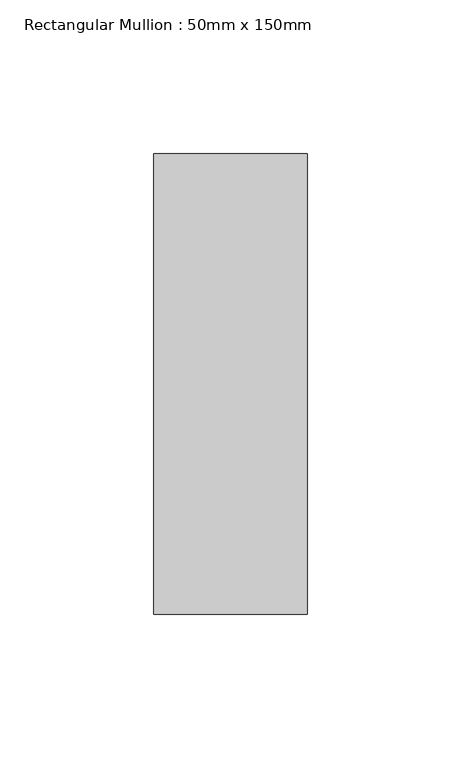
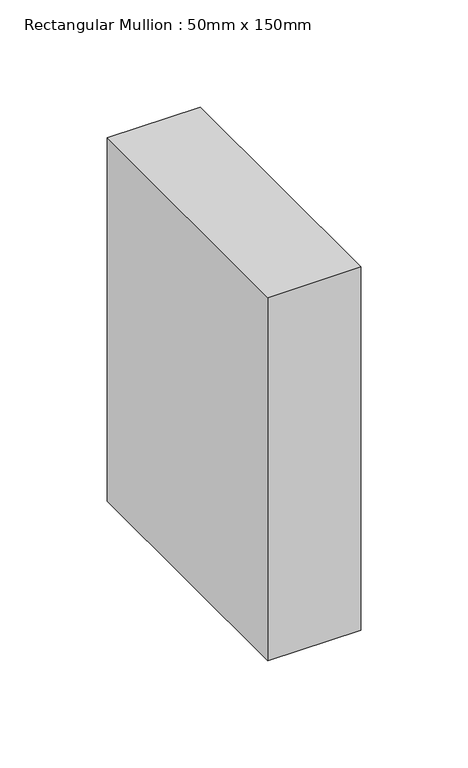
"""IFC4 building model written with IfcOpenShell, lengths in millimetres: member geometry, Rectangular Mullion : 50mm x 150mm."""

from ifc_helpers import new_model, si_unit, frame, origin, place, context, project, spatial, polyline, outline, extrude, source, transform, mapped, element, save


def rectangular_mullion_50mm_x_150mm_a0b84712(model_context):
    return source(origin(), model_context, "Body", "SweptSolid", [
        extrude(outline(polyline([(0.0, 75.0), (0.0, -75.0), (-50.0, -75.0), (-50.0, 75.0), (0.0, 75.0)])), frame((0.0, 0.0, -206.8181818), z_axis=(0.0, 0.0, 1.0), x_axis=(1.0, 0.0, 0.0)), (0.0, 0.0, 1.0), 206.8181818),
    ])


if __name__ == "__main__":
    model = new_model("IFC4")
    model_context = context("Model", 3, world=origin())
    ifc_project = project(units=[si_unit("LENGTHUNIT", "METRE", prefix="MILLI")], contexts=[model_context])
    site = spatial("IfcSite", under=ifc_project)
    building = spatial("IfcBuilding", under=site)
    placement = place(None, origin())
    rectangular_mullion_50mm_x_150mm_shape = rectangular_mullion_50mm_x_150mm_a0b84712(model_context)
    element("IfcMember", 1, ObjectType="Rectangular Mullion : 50mm x 150mm", at=placement, inside=building, context=model_context, shape_type="MappedRepresentation", body=[
        mapped(rectangular_mullion_50mm_x_150mm_shape, transform((0.0, 0.0, 0.0), x_axis=(1.0, 0.0, 0.0), y_axis=(0.0, 1.0, 0.0), z_axis=(0.0, 0.0, 1.0))),
    ])
    save(model, "model.ifc")

# Revit data of these elements
# Type "Rectangular Mullion : 50mm x 150mm"
#   built-in parameter 1007304 = 0.492126 (stored number, unit not read)
#   built-in parameter 1007301 = 0.082021 (stored number, unit not read)
#   built-in parameter 1007300 = 0.082021 (stored number, unit not read)
# Element 1 (IfcMember, "Rectangular Mullion : 50mm x 150mm")
#   Materials on its faces: "Aluminum"
# Materials
#   "Aluminum": class "Metal", colour RGB 244 244 244, transparency 0, Description = "Aluminum 6061", Cost = 0
